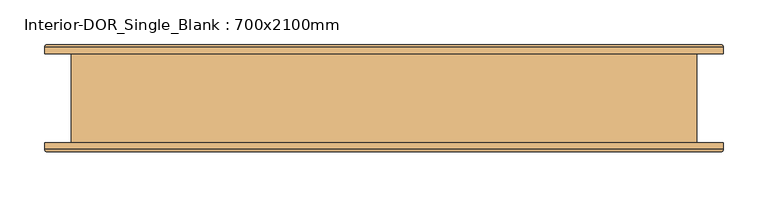
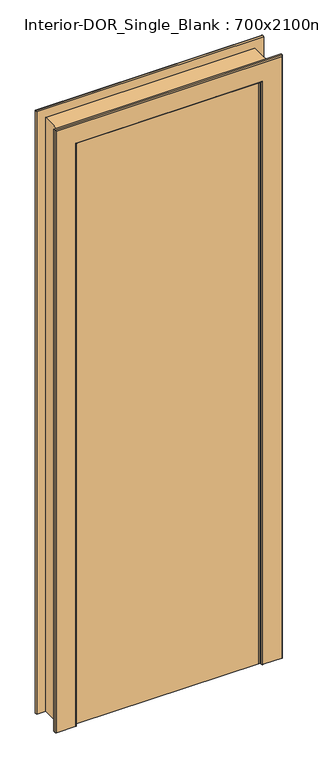
"""IFC4 building model written with IfcOpenShell, lengths in millimetres: door geometry, Interior-DOR_Single_Blank : 700x2100mm."""

from ifc_helpers import new_model, si_unit, frame, origin, origin_with_axes, place, context, project, spatial, polyline, circle_curve, ellipse_curve, outline, extrude, faceted_brep, source, transform, mapped, element, save
from ifc_brep_helpers import plane_surface, cylinder_surface, advanced_brep


def interior_dor_single_blank_700x2100mm_7bd7bfec(model_context):
    return source(origin(), model_context, "Body", "SolidModel", [
        advanced_brep(
        [(-310.0, -50.0, 0.0), (-310.0, -57.0, 0.0), (-313.0, -60.0, 0.0), (-377.0, -60.0, 0.0), (-380.0, -57.0, 0.0), (-380.0, -50.0, 0.0), (-310.0, -50.0, 2060.0), (-310.0, -57.0, 2060.0), (-313.0, -60.0, 2063.0), (313.0, -60.0, 2063.0), (313.0, -60.0, 0.0), (377.0, -60.0, 0.0), (377.0, -60.0, 2127.0), (-377.0, -60.0, 2127.0), (-380.0, -57.0, 2130.0), (-380.0, -50.0, 2130.0), (380.0, -50.0, 2130.0), (380.0, -50.0, 0.0), (310.0, -50.0, 0.0), (310.0, -50.0, 2060.0), (310.0, -57.0, 2060.0), (310.0, -57.0, 0.0), (380.0, -57.0, 0.0), (380.0, -57.0, 2130.0)],
        [
            (0, 1),
            (1, 2, circle_curve(frame((-313.0, -57.0, 0.0), z_axis=(0.0, 0.0, -1.0), x_axis=(-1.0, 0.0, 0.0)), 3.0)),
            (2, 3),
            (3, 4, circle_curve(frame((-377.0, -57.0, 0.0), z_axis=(0.0, 0.0, -1.0), x_axis=(-1.0, 0.0, 0.0)), 3.0)),
            (4, 5),
            (5, 0),
            (0, 6),
            (6, 7),
            (7, 1),
            (7, 8, ellipse_curve(frame((-313.0, -57.0, 2063.0), z_axis=(-0.7071067811865475, 0.0, -0.7071067811865475), x_axis=(0.7071067811865474, 0.0, -0.7071067811865476)), 4.2426407, 3.0)),
            (8, 2),
            (8, 9),
            (9, 10),
            (10, 11),
            (11, 12),
            (12, 13),
            (13, 3),
            (13, 14, ellipse_curve(frame((-377.0, -57.0, 2127.0), z_axis=(-0.7071067811865475, 0.0, -0.7071067811865475), x_axis=(0.7071067811865474, 0.0, -0.7071067811865476)), 4.2426407, 3.0)),
            (14, 4),
            (14, 15),
            (15, 5),
            (15, 16),
            (16, 17),
            (17, 18),
            (18, 19),
            (19, 6),
            (9, 20, ellipse_curve(frame((313.0, -57.0, 2063.0), z_axis=(0.7071067811865475, 0.0, -0.7071067811865475), x_axis=(0.7071067811865474, 0.0, 0.7071067811865476)), 4.2426407, 3.0)),
            (20, 21),
            (21, 10, circle_curve(frame((313.0, -57.0, 0.0), z_axis=(0.0, 0.0, 1.0), x_axis=(1.0, 0.0, 0.0)), 3.0)),
            (17, 22),
            (22, 11, circle_curve(frame((377.0, -57.0, 0.0), z_axis=(0.0, 0.0, -1.0), x_axis=(1.0, 0.0, 0.0)), 3.0)),
            (21, 18),
            (23, 12, ellipse_curve(frame((377.0, -57.0, 2127.0), z_axis=(0.7071067811865475, 0.0, -0.7071067811865475), x_axis=(0.7071067811865474, 0.0, 0.7071067811865476)), 4.2426407, 3.0)),
            (22, 23),
            (16, 23),
            (20, 19),
            (20, 7),
            (23, 14),
        ],
        [
            plane_surface(frame((-350.0, 50.0, 0.0), z_axis=(0.0, 0.0, -1.0), x_axis=(0.0, -1.0, 0.0))),
            plane_surface(frame((-310.0, -50.0, 0.0), z_axis=(1.0, 0.0, 0.0), x_axis=(0.0, 0.0, 1.0))),
            cylinder_surface(frame((-313.0, -57.0, 0.0), z_axis=(0.0, 0.0, -1.0), x_axis=(-1.0, 0.0, 0.0)), 3.0),
            plane_surface(frame((-313.0, -60.0, 0.0), z_axis=(0.0, -1.0, 0.0), x_axis=(0.0, 0.0, 1.0))),
            cylinder_surface(frame((-377.0, -57.0, 0.0), z_axis=(0.0, 0.0, -1.0), x_axis=(-1.0, 0.0, 0.0)), 3.0),
            plane_surface(frame((-380.0, -57.0, 0.0), z_axis=(-1.0, 0.0, 0.0), x_axis=(0.0, 0.0, 1.0))),
            plane_surface(frame((-380.0, -50.0, 0.0), z_axis=(0.0, 1.0, 0.0), x_axis=(0.0, 0.0, 1.0))),
            cylinder_surface(frame((313.0, -57.0, 2100.0), z_axis=(0.0, 0.0, 1.0), x_axis=(1.0, 0.0, 0.0)), 3.0),
            plane_surface(frame((350.0, 50.0, 0.0), z_axis=(0.0, 0.0, -1.0), x_axis=(0.0, -1.0, 0.0))),
            cylinder_surface(frame((377.0, -57.0, 2100.0), z_axis=(0.0, 0.0, 1.0), x_axis=(1.0, 0.0, 0.0)), 3.0),
            plane_surface(frame((380.0, -57.0, 2130.0), z_axis=(1.0, 0.0, 0.0), x_axis=(0.0, 0.0, -1.0))),
            plane_surface(frame((310.0, -50.0, 2060.0), z_axis=(-1.0, 0.0, 0.0), x_axis=(0.0, 0.0, -1.0))),
            plane_surface(frame((-310.0, -50.0, 2060.0), z_axis=(0.0, 0.0, -1.0), x_axis=(1.0, 0.0, 0.0))),
            cylinder_surface(frame((-350.0, -57.0, 2063.0), z_axis=(-1.0, 0.0, 0.0), x_axis=(0.0, 0.0, 1.0)), 3.0),
            cylinder_surface(frame((-350.0, -57.0, 2127.0), z_axis=(-1.0, 0.0, 0.0), x_axis=(0.0, 0.0, 1.0)), 3.0),
            plane_surface(frame((-380.0, -57.0, 2130.0), z_axis=(0.0, 0.0, 1.0), x_axis=(1.0, 0.0, 0.0))),
        ],
        [
            (0, [[1, 2, 3, 4, 5, 6]]),
            (1, [[-1, 7, 8, 9]]),
            (2, [[-2, -9, 10, 11]]),
            (3, [[-3, -11, 12, 13, 14, 15, 16, 17]]),
            (4, [[-4, -17, 18, 19]]),
            (5, [[-5, -19, 20, 21]]),
            (6, [[-6, -21, 22, 23, 24, 25, 26, -7]]),
            (7, [[27, 28, 29, -13]]),
            (8, [[-24, 30, 31, -14, -29, 32]]),
            (9, [[33, -15, -31, 34]]),
            (10, [[35, -34, -30, -23]]),
            (11, [[36, -25, -32, -28]]),
            (12, [[-8, -26, -36, 37]]),
            (13, [[-10, -37, -27, -12]]),
            (14, [[-18, -16, -33, 38]]),
            (15, [[-20, -38, -35, -22]]),
        ],
    ),
        advanced_brep(
        [(-380.0, 50.0, 0.0), (-380.0, 57.0, 0.0), (-377.0, 60.0, 0.0), (-313.0, 60.0, 0.0), (-310.0, 57.0, 0.0), (-310.0, 50.0, 0.0), (-380.0, 50.0, 2130.0), (-380.0, 57.0, 2130.0), (-377.0, 60.0, 2127.0), (377.0, 60.0, 2127.0), (377.0, 60.0, 0.0), (313.0, 60.0, 0.0), (313.0, 60.0, 2063.0), (-313.0, 60.0, 2063.0), (-310.0, 57.0, 2060.0), (-310.0, 50.0, 2060.0), (310.0, 50.0, 2060.0), (310.0, 50.0, 0.0), (380.0, 50.0, 0.0), (380.0, 50.0, 2130.0), (380.0, 57.0, 2130.0), (380.0, 57.0, 0.0), (310.0, 57.0, 0.0), (310.0, 57.0, 2060.0)],
        [
            (0, 1),
            (1, 2, circle_curve(frame((-377.0, 57.0, 0.0), z_axis=(0.0, 0.0, -1.0), x_axis=(-1.0, 0.0, 0.0)), 3.0)),
            (2, 3),
            (3, 4, circle_curve(frame((-313.0, 57.0, 0.0), z_axis=(0.0, 0.0, -1.0), x_axis=(-1.0, 0.0, 0.0)), 3.0)),
            (4, 5),
            (5, 0),
            (0, 6),
            (6, 7),
            (7, 1),
            (7, 8, ellipse_curve(frame((-377.0, 57.0, 2127.0), z_axis=(-0.7071067811865475, 0.0, -0.7071067811865475), x_axis=(0.7071067811865474, 0.0, -0.7071067811865476)), 4.2426407, 3.0)),
            (8, 2),
            (8, 9),
            (9, 10),
            (10, 11),
            (11, 12),
            (12, 13),
            (13, 3),
            (13, 14, ellipse_curve(frame((-313.0, 57.0, 2063.0), z_axis=(-0.7071067811865475, 0.0, -0.7071067811865475), x_axis=(0.7071067811865474, 0.0, -0.7071067811865476)), 4.2426407, 3.0)),
            (14, 4),
            (14, 15),
            (15, 5),
            (15, 16),
            (16, 17),
            (17, 18),
            (18, 19),
            (19, 6),
            (9, 20, ellipse_curve(frame((377.0, 57.0, 2127.0), z_axis=(0.7071067811865475, 0.0, -0.7071067811865475), x_axis=(0.7071067811865474, 0.0, 0.7071067811865476)), 4.2426407, 3.0)),
            (20, 21),
            (21, 10, circle_curve(frame((377.0, 57.0, 0.0), z_axis=(0.0, 0.0, 1.0), x_axis=(1.0, 0.0, 0.0)), 3.0)),
            (17, 22),
            (22, 11, circle_curve(frame((313.0, 57.0, 0.0), z_axis=(0.0, 0.0, -1.0), x_axis=(1.0, 0.0, 0.0)), 3.0)),
            (21, 18),
            (23, 12, ellipse_curve(frame((313.0, 57.0, 2063.0), z_axis=(0.7071067811865475, 0.0, -0.7071067811865475), x_axis=(0.7071067811865474, 0.0, 0.7071067811865476)), 4.2426407, 3.0)),
            (22, 23),
            (16, 23),
            (20, 19),
            (20, 7),
            (23, 14),
        ],
        [
            plane_surface(frame((-350.0, 50.0, 0.0), z_axis=(0.0, 0.0, -1.0), x_axis=(0.0, -1.0, 0.0))),
            plane_surface(frame((-380.0, 50.0, 0.0), z_axis=(-1.0, 0.0, 0.0), x_axis=(0.0, 0.0, 1.0))),
            cylinder_surface(frame((-377.0, 57.0, 0.0), z_axis=(0.0, 0.0, -1.0), x_axis=(-1.0, 0.0, 0.0)), 3.0),
            plane_surface(frame((-377.0, 60.0, 0.0), z_axis=(0.0, 1.0, 0.0), x_axis=(0.0, 0.0, 1.0))),
            cylinder_surface(frame((-313.0, 57.0, 0.0), z_axis=(0.0, 0.0, -1.0), x_axis=(-1.0, 0.0, 0.0)), 3.0),
            plane_surface(frame((-310.0, 57.0, 0.0), z_axis=(1.0, 0.0, 0.0), x_axis=(0.0, 0.0, 1.0))),
            plane_surface(frame((-310.0, 50.0, 0.0), z_axis=(0.0, -1.0, 0.0), x_axis=(0.0, 0.0, 1.0))),
            cylinder_surface(frame((377.0, 57.0, 2100.0), z_axis=(0.0, 0.0, 1.0), x_axis=(1.0, 0.0, 0.0)), 3.0),
            plane_surface(frame((350.0, 50.0, 0.0), z_axis=(0.0, 0.0, -1.0), x_axis=(0.0, -1.0, 0.0))),
            cylinder_surface(frame((313.0, 57.0, 2100.0), z_axis=(0.0, 0.0, 1.0), x_axis=(1.0, 0.0, 0.0)), 3.0),
            plane_surface(frame((310.0, 57.0, 2060.0), z_axis=(-1.0, 0.0, 0.0), x_axis=(0.0, 0.0, -1.0))),
            plane_surface(frame((380.0, 50.0, 2130.0), z_axis=(1.0, 0.0, 0.0), x_axis=(0.0, 0.0, -1.0))),
            plane_surface(frame((-380.0, 50.0, 2130.0), z_axis=(0.0, 0.0, 1.0), x_axis=(1.0, 0.0, 0.0))),
            cylinder_surface(frame((-350.0, 57.0, 2127.0), z_axis=(-1.0, 0.0, 0.0), x_axis=(0.0, 0.0, 1.0)), 3.0),
            cylinder_surface(frame((-350.0, 57.0, 2063.0), z_axis=(-1.0, 0.0, 0.0), x_axis=(0.0, 0.0, 1.0)), 3.0),
            plane_surface(frame((-310.0, 57.0, 2060.0), z_axis=(0.0, 0.0, -1.0), x_axis=(1.0, 0.0, 0.0))),
        ],
        [
            (0, [[1, 2, 3, 4, 5, 6]]),
            (1, [[-1, 7, 8, 9]]),
            (2, [[-2, -9, 10, 11]]),
            (3, [[-3, -11, 12, 13, 14, 15, 16, 17]]),
            (4, [[-4, -17, 18, 19]]),
            (5, [[-5, -19, 20, 21]]),
            (6, [[-6, -21, 22, 23, 24, 25, 26, -7]]),
            (7, [[27, 28, 29, -13]]),
            (8, [[-24, 30, 31, -14, -29, 32]]),
            (9, [[33, -15, -31, 34]]),
            (10, [[35, -34, -30, -23]]),
            (11, [[36, -25, -32, -28]]),
            (12, [[-8, -26, -36, 37]]),
            (13, [[-10, -37, -27, -12]]),
            (14, [[-18, -16, -33, 38]]),
            (15, [[-20, -38, -35, -22]]),
        ],
    ),
        faceted_brep([(-350.0, 50.0, 0.0), (-305.0, 50.0, 0.0), (-305.0, 35.0, 0.0), (-285.0, 35.0, 0.0), (-285.0, -5.0, 0.0), (-305.0, -5.0, 0.0), (-305.0, -50.0, 0.0), (-350.0, -50.0, 0.0), (-350.0, 50.0, 2100.0), (350.0, 50.0, 2100.0), (350.0, 50.0, 0.0), (305.0, 50.0, 0.0), (305.0, 50.0, 2055.0), (-305.0, 50.0, 2055.0), (-305.0, 35.0, 2055.0), (305.0, 35.0, 2055.0), (305.0, 35.0, 0.0), (285.0, 35.0, 0.0), (285.0, 35.0, 2035.0), (-285.0, 35.0, 2035.0), (-285.0, -5.0, 2035.0), (285.0, -5.0, 2035.0), (285.0, -5.0, 0.0), (305.0, -5.0, 0.0), (305.0, -5.0, 2055.0), (-305.0, -5.0, 2055.0), (-305.0, -50.0, 2055.0), (305.0, -50.0, 2055.0), (305.0, -50.0, 0.0), (350.0, -50.0, 0.0), (350.0, -50.0, 2100.0), (-350.0, -50.0, 2100.0)], [[[0, 1, 2, 3, 4, 5, 6, 7]], [[1, 0, 8, 9, 10, 11, 12, 13]], [[2, 1, 13, 14]], [[3, 2, 14, 15, 16, 17, 18, 19]], [[4, 3, 19, 20]], [[5, 4, 20, 21, 22, 23, 24, 25]], [[6, 5, 25, 26]], [[7, 6, 26, 27, 28, 29, 30, 31]], [[0, 7, 31, 8]], [[9, 30, 29, 10]], [[10, 29, 28, 23, 22, 17, 16, 11]], [[15, 12, 11, 16]], [[21, 18, 17, 22]], [[27, 24, 23, 28]], [[20, 19, 18, 21]], [[26, 25, 24, 27]], [[8, 31, 30, 9]], [[14, 13, 12, 15]]]),
        extrude(outline(polyline([(305.0, -50.0), (-305.0, -50.0), (-305.0, -5.0), (305.0, -5.0), (305.0, -50.0)])), origin_with_axes(), (0.0, 0.0, 1.0), 2055.0),
    ])


if __name__ == "__main__":
    model = new_model("IFC4")
    model_context = context("Model", 3, world=origin())
    ifc_project = project(units=[si_unit("LENGTHUNIT", "METRE", prefix="MILLI")], contexts=[model_context])
    site = spatial("IfcSite", under=ifc_project)
    building = spatial("IfcBuilding", under=site)
    placement = place(None, origin())
    interior_dor_single_blank_700x2100mm_shape = interior_dor_single_blank_700x2100mm_7bd7bfec(model_context)
    element("IfcDoor", 1, ObjectType="Interior-DOR_Single_Blank : 700x2100mm", at=placement, inside=building, context=model_context, shape_type="MappedRepresentation", body=[
        mapped(interior_dor_single_blank_700x2100mm_shape, transform((0.0, 0.0, 0.0), x_axis=(1.0, 0.0, 0.0), y_axis=(0.0, 1.0, 0.0), z_axis=(0.0, 0.0, 1.0))),
    ])
    save(model, "model.ifc")

# Revit data of these elements
# Type "Interior-DOR_Single_Blank : 700x2100mm"
#   Type IfcGUID = "1sWU2cMPP4xwRoAc3TXQKN"
#   Assembly Code = "C1020120"
#   Type Mark = "196"
#   Classification.Uniclass.EF.Number = "EF_25_30"
#   Classification.Uniclass.EF.Description = "Doors and windows"
#   WindLoadRating = "n/a"
#   WaterTightnessRating = "n/a"
#   WarrantyStartDate [instance default] = "1900-12-31T23:59:59"
#   WarrantyGuarantorParts = "n/a"
#   WarrantyGuarantorLabor = "n/a"
#   WarrantyDurationUnit = "year"
#   WarrantyDurationParts = "n/a"
#   WarrantyDurationLabor = "n/a"
#   WarrantyDescription = "n/a"
#   Version = "2"
#   Uniclass2015Version = "Systems v1.9"
#   Uniclass2015Title = "Doorset systems"
#   Uniclass2015Code = "Ss_25_30_20_25"
#   URL = "www.nationalbimlibrary.com"
#   TagNumber [instance default] = "n/a"
#   SustainabilityPerformance = "n/a"
#   Status = "UNSET"
#   Size = "1010 x 2100 mm"
#   Shape = "n/a"
#   SerialNumber [instance default] = "n/a"
#   SecurityRating = "n/a"
#   Revision = "n/a"
#   ReplacementCost = "n/a"
#   Reference = "n/a"
#   ProductInformation = "n/a"
#   Operation = "SINGLE_SWING_RIGHT"
#   OmniClassVersion = "Table 22 2012-05-16"
#   OmniClassTitle = "Doors and Frames"
#   OmniClassCode = "22-08 10 00"
#   Name = "DoorsetSystem_Interior-Single_Blank"
#   NBSReference = "25-50-20/120"
#   NBSDescription = "Doorset system"
#   NBSCertification = "www.nationalbimlibrary.com/cert/mlf45nxc"
#   ModelReference = "Interior Single Door"
#   ModelNumber = "n/a"
#   Model = "Interior Single Door"
#   MechanicalLoadRating = "n/a"
#   Material = "n/a"
#   ManufacturerURL = "n/a"
#   ManufacturerName = "n/a"
#   Manufacturer = "info@theNBS.com"
#   InstallationDate [instance default] = "1900-12-31T23:59:59"
#   IfcExportType = "DOOR"
#   IfcExportAs = "IfcDoorType"
#   HygrothermalRating = "n/a"
#   Grade = "n/a"
#   FireRating = "n/a"
#   Fire Rating = "n/a"
#   Finish = "n/a"
#   Features = "n/a"
#   ExpectedLife = "n/a"
#   DurationUnit = "n/a"
#   DurabilityRating = "n/a"
#   DoorNumber [instance default] = "n/a"
#   Description = "Generic single interior door"
#   Construction Type = "USERDEFINED"
#   Constituents = "n/a"
#   ComponentNumber [instance default] = "n/a"
#   Color = "n/a"
#   CodePerformance = "n/a"
#   Category = "Ss_25_30_20_25:Doorset systems"
#   BarCode [instance default] = "n/a"
#   BIMObjectName = "NBS_DoorsetSystem_Interior-Single_Blank"
#   Author = "NBS"
#   AssetType = "Fixed"
#   AssetIdentifier [instance default] = "n/a"
#   AcousticRating = "n/a"
#   AccessibilityPerformance = "n/a"
#   Width = 0.7 m
#   WallThickness [instance default] = 0.15 m
#   ThresholdHeight = 0.015 m
#   Thickness = 0.15 m
#   ThermalTransmittance = 0
#   StructuralToleranceJamb = 0 m
#   StructuralToleranceHead = 0 m
#   StructuralOpeningWidth = 0.7 m
#   StructuralOpeningHeight = 2.1 m
#   StopProjection = 0.02 m
#   StopDepth = 0.04 m
#   Rough Width [instance default] = 0.7 m
#   Rough Height [instance default] = 2.1 m
#   RebateDepth = 0.045 m
#   PanelWidth = 0.61 m
#   PanelUndercut = 0 m
#   PanelHeight = 2.055 m
#   PanelDepth = 0.045 m
#   OpeningTolerance = 0 m
#   NominalWidth = 0.7 m
#   NominalLength = 0 m
#   NominalHeight = 2.1 m
#   Infiltration = 0
#   Height = 2.1 m
#   GlazingAreaFraction = 0
#   FrameThickness = 0.045 m
#   FrameSetback [instance default] = 0 m
#   FrameDepth [instance default] = 0.15 m
#   FinishThicknessInternal [instance default] = 0 m
#   FinishThicknessExternal [instance default] = 0 m
#   ClearOpeningWidth = 0.57 m
#   ClearOpeningHeight = 2.035 m
#   CalculatedInteriorVoidDepth [instance default] = 0.3 m
#   ArchitraveWidth = 0.07 m
#   ArchitraveThickness = 0.01 m
#   ArchitraveSetbackFromFrameFace = 0.005 m
#   SmokeStop = no
#   SingleRebate = no
#   SelfClosing = no
#   PlantedStop = yes
#   IsExternal = no
#   HasDrive = no
#   HandicapAccessible = no
#   Wall Closure = 4
#   FireExit = no
#   ArchitraveFrontRequired [instance default] = yes
#   ArchitraveBackRequired [instance default] = yes
#   PanelMaterial = NBS_Concept
#   HardwareFinish = NBS_Concept
#   FrameSectionMaterial = NBS_Concept
#   Function = (empty or 0)
#   Cost = 0
# Element 1 (IfcDoor, "Interior-DOR_Single_Blank : 700x2100mm")
#   WallThickness = 0.1 m
#   FrameDepth = 0.1 m
#   Materials on its faces: "NBS_Concept"
# Materials
#   "NBS_Concept": class "Generic", colour RGB 255 255 255, transparency 0, Description = "To be specified", Cost = 0
